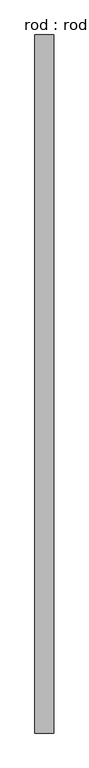
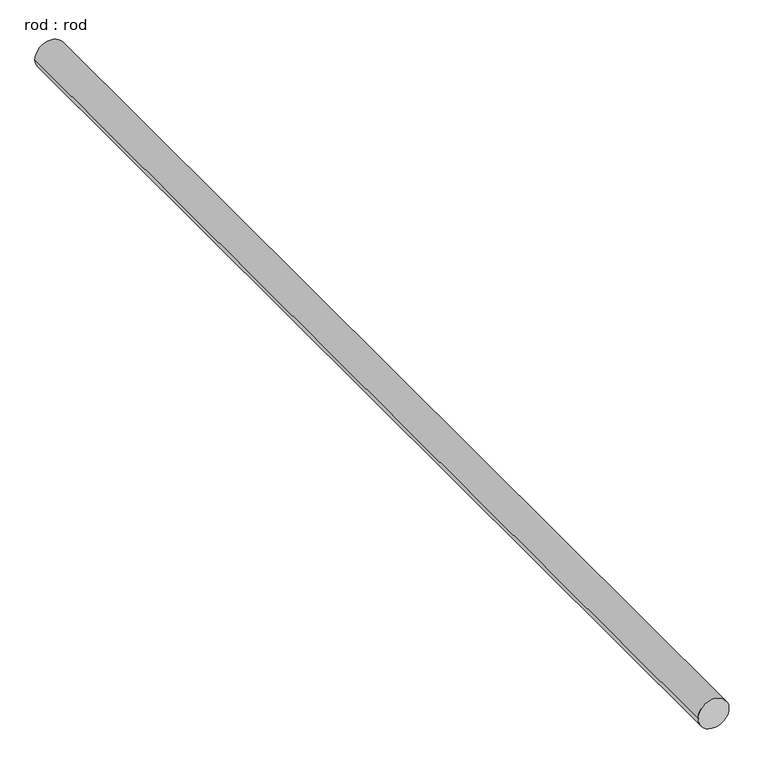
"""IFC4 building model written with IfcOpenShell, lengths in millimetres: proxy geometry, rod : rod."""

import ifcopenshell
import ifcopenshell.guid

model = None  # the IFC model being written
_history = None  # IfcOwnerHistory: only IFC2X3 demands one
_inside = {}  # id of a spatial element -> (the spatial element, [elements in it])
_under = {}  # id of a project, library or spatial element -> (it, [spatial elements below it])
_declared = {}  # id of a project -> (the project, [libraries it declares])
_typed = {}  # id of a type object -> (the type object, [elements of that type])
_made_of = {}  # id of a material, layer set ... -> (it, [elements and type objects made of it])


def new_model(schema):
    """Start an empty IFC model of exactly this schema.

    Asked for "IFC4X3", IfcOpenShell would pick the latest addendum, in which some entities
    have other attributes; the version numbers below select the first issue.
    IFC2X3 requires an IfcOwnerHistory on every rooted entity: one is made here for all.
    """
    global model, _history
    if schema == "IFC4X3":
        model = ifcopenshell.file(schema_version=(4, 3, 0, 0))
    else:
        model = ifcopenshell.file(schema=schema)
    _inside.clear()
    _under.clear()
    _declared.clear()
    _typed.clear()
    _made_of.clear()
    _history = None
    if model.schema == "IFC2X3":
        org = make("IfcOrganization", Name="unknown")
        user = make(
            "IfcPersonAndOrganization",
            ThePerson=make("IfcPerson", FamilyName="unknown"),
            TheOrganization=org,
        )
        app = make(
            "IfcApplication",
            ApplicationDeveloper=org,
            Version="unknown",
            ApplicationFullName="unknown",
            ApplicationIdentifier="unknown",
        )
        _history = make(
            "IfcOwnerHistory",
            OwningUser=user,
            OwningApplication=app,
            ChangeAction="ADDED",
            CreationDate=0,
        )
    return model


def make(cls, **values):
    """One entity of the class cls with the attributes given. An attribute that is None is left unset."""
    return model.create_entity(
        cls, **{name: value for name, value in values.items() if value is not None}
    )


def rooted(cls, **values):
    """An entity with a GlobalId (a new one), such as an element, a storey or a relation."""
    return make(cls, GlobalId=ifcopenshell.guid.new(), OwnerHistory=_history, **values)


def si_unit(unit_type, name, prefix=None):
    """IfcSIUnit, for example si_unit("LENGTHUNIT", "METRE", prefix="MILLI")."""
    return make("IfcSIUnit", UnitType=unit_type, Prefix=prefix, Name=name)


def assignment(units):
    """IfcUnitAssignment: the units of a project."""
    return None if units is None else make("IfcUnitAssignment", Units=units)


def point(xyz):
    """IfcCartesianPoint."""
    return None if xyz is None else make("IfcCartesianPoint", Coordinates=xyz)


def direction(xyz):
    """IfcDirection."""
    return None if xyz is None else make("IfcDirection", DirectionRatios=xyz)


def frame(location, z_axis=None, x_axis=None):
    """IfcAxis2Placement3D, a coordinate frame: its origin and axes. An axis left out is left unset."""
    return make(
        "IfcAxis2Placement3D",
        Location=point(location),
        Axis=direction(z_axis),
        RefDirection=direction(x_axis),
    )


def frame_2d(location, x_axis=None):
    """IfcAxis2Placement2D, a coordinate frame in the plane: its origin and x axis."""
    return make(
        "IfcAxis2Placement2D", Location=point(location), RefDirection=direction(x_axis)
    )


def origin():
    """The frame at (0, 0, 0) with its axes left unset."""
    return frame((0.0, 0.0, 0.0))


def place(relative_to, where):
    """IfcLocalPlacement: puts the frame where relative to a parent placement (None: the world)."""
    return make(
        "IfcLocalPlacement", PlacementRelTo=relative_to, RelativePlacement=where
    )


def context(
    kind, dimensions, precision=None, world=None, true_north=None, identifier=None
):
    """IfcGeometricRepresentationContext, for example the 3D "Model" context."""
    return make(
        "IfcGeometricRepresentationContext",
        ContextIdentifier=identifier,
        ContextType=kind,
        CoordinateSpaceDimension=dimensions,
        Precision=precision,
        WorldCoordinateSystem=world,
        TrueNorth=true_north,
    )


def project(units=None, contexts=None):
    """IfcProject with its units and contexts."""
    return rooted(
        "IfcProject",
        Name="project",
        RepresentationContexts=contexts,
        UnitsInContext=assignment(units),
    )


def spatial(cls, under=None, at=None, **own):
    """A site, building, storey or space (cls), placed at a placement, below another one or the project."""
    s = rooted(cls, ObjectPlacement=at, **own)
    if under is not None:
        _under.setdefault(under.id(), (under, []))[1].append(s)
    return s


def circle_curve(where, radius):
    """IfcCircle in the frame where."""
    return make("IfcCircle", Position=where, Radius=radius)


def trimmed(basis, trim1, trim2, sense, master):
    """IfcTrimmedCurve: the piece of a basis curve between two trims."""
    return make(
        "IfcTrimmedCurve",
        BasisCurve=basis,
        Trim1=trim1,
        Trim2=trim2,
        SenseAgreement=sense,
        MasterRepresentation=master,
    )


def segment(curve, same_sense, transition):
    """IfcCompositeCurveSegment."""
    return make(
        "IfcCompositeCurveSegment",
        Transition=transition,
        SameSense=same_sense,
        ParentCurve=curve,
    )


def composite_curve(segments, self_intersect=None):
    """IfcCompositeCurve: segments joined end to end."""
    return make("IfcCompositeCurve", Segments=segments, SelfIntersect=self_intersect)


def outline(outer, holes=None, kind="AREA"):
    """IfcArbitraryClosedProfileDef: a profile drawn as a closed curve; with holes, ...WithVoids."""
    if holes is None:
        return make("IfcArbitraryClosedProfileDef", ProfileType=kind, OuterCurve=outer)
    return make(
        "IfcArbitraryProfileDefWithVoids",
        ProfileType=kind,
        OuterCurve=outer,
        InnerCurves=holes,
    )


def extrude(swept, where, along, depth):
    """IfcExtrudedAreaSolid: the profile swept, set in the frame where, extruded along a direction by depth."""
    return make(
        "IfcExtrudedAreaSolid",
        SweptArea=swept,
        Position=where,
        ExtrudedDirection=direction(along),
        Depth=depth,
    )


def shape(context_of_items, identifier, shape_type, items):
    """IfcShapeRepresentation: the items that make up one representation, for example the "Body"."""
    return make(
        "IfcShapeRepresentation",
        ContextOfItems=context_of_items,
        RepresentationIdentifier=identifier,
        RepresentationType=shape_type,
        Items=items,
    )


def source(mapping_origin, context_of_items, identifier, shape_type, items):
    """IfcRepresentationMap: a shape defined once, which mapped items show again and again."""
    return make(
        "IfcRepresentationMap",
        MappingOrigin=mapping_origin,
        MappedRepresentation=shape(context_of_items, identifier, shape_type, items),
    )


def transform(
    local_origin,
    x_axis=None,
    y_axis=None,
    z_axis=None,
    scale=None,
    scale2=None,
    scale3=None,
    uniform=True,
):
    """IfcCartesianTransformationOperator3D, or its non-uniform kind. x_axis, y_axis, z_axis: its Axis1, 2, 3."""
    if uniform:
        return make(
            "IfcCartesianTransformationOperator3D",
            Axis1=direction(x_axis),
            Axis2=direction(y_axis),
            LocalOrigin=point(local_origin),
            Scale=scale,
            Axis3=direction(z_axis),
        )
    return make(
        "IfcCartesianTransformationOperator3DnonUniform",
        Axis1=direction(x_axis),
        Axis2=direction(y_axis),
        LocalOrigin=point(local_origin),
        Scale=scale,
        Axis3=direction(z_axis),
        Scale2=scale2,
        Scale3=scale3,
    )


def mapped(mapping_source, mapping_target):
    """IfcMappedItem: shows the shape of a source again, moved by a transform."""
    return make(
        "IfcMappedItem", MappingSource=mapping_source, MappingTarget=mapping_target
    )


def made_of(thing, what):
    """Note that an element or type object is made of a material, layer set ...; save() writes the relation."""
    if what is not None:
        _made_of.setdefault(what.id(), (what, []))[1].append(thing)
    return thing


def element(
    cls,
    number,
    at=None,
    inside=None,
    cuts=None,
    type_object=None,
    material=None,
    context=None,
    identifier="Body",
    shape_type=None,
    held_by="IfcProductDefinitionShape",
    body=None,
    shapes=None,
    **own,
):
    """One element of the class cls, such as IfcWall. Its Tag is "e" and its number.

    at: its placement. inside: the storey or other place that contains it. cuts: it is an
    opening in that element (IfcRelVoidsElement). A single representation is given by context,
    identifier, shape_type and body (its items); several are given by shapes. held_by: the class
    of the entity that holds the representations. save() writes the other relations.
    """
    e = rooted(cls, Tag="e%d" % number, ObjectPlacement=at, **own)
    if body is not None:
        shapes = [shape(context, identifier, shape_type, body)]
    if shapes is not None:
        e.Representation = make(held_by, Representations=shapes)
    if inside is not None:
        _inside.setdefault(inside.id(), (inside, []))[1].append(e)
    if cuts is not None:
        rooted(
            "IfcRelVoidsElement", RelatingBuildingElement=cuts, RelatedOpeningElement=e
        )
    if type_object is not None:
        _typed.setdefault(type_object.id(), (type_object, []))[1].append(e)
    return made_of(e, material)


def aggregate(whole, parts):
    """IfcRelAggregates: a whole, such as a stair, and the parts it consists of."""
    return rooted("IfcRelAggregates", RelatingObject=whole, RelatedObjects=parts)


def save(model, path):
    """Write the relations noted so far, then the file.

    IfcRelAggregates (storeys below a building ...), IfcRelContainedInSpatialStructure (elements
    in a storey), IfcRelDefinesByType, IfcRelAssociatesMaterial and IfcRelDeclares: one each for
    every whole, place, type object, material and project.
    """
    for whole, parts in _under.values():
        aggregate(whole, parts)
    for where, things in _inside.values():
        rooted(
            "IfcRelContainedInSpatialStructure",
            RelatedElements=things,
            RelatingStructure=where,
        )
    for kind, things in _typed.values():
        rooted("IfcRelDefinesByType", RelatedObjects=things, RelatingType=kind)
    for what, things in _made_of.values():
        rooted("IfcRelAssociatesMaterial", RelatedObjects=things, RelatingMaterial=what)
    for by, libraries in _declared.values():
        rooted("IfcRelDeclares", RelatingContext=by, RelatedDefinitions=libraries)
    model.write(path)


def rod_rod_d696530c(model_context):
    return source(origin(), model_context, "Body", "SweptSolid", [
        extrude(outline(composite_curve([segment(trimmed(circle_curve(frame_2d((0.0108462, 0.0)), 200.0), [point((0.0108462, 200.0))], [point((0.0108462, -200.0))], False, "CARTESIAN"), True, "CONTINUOUS"), segment(trimmed(circle_curve(frame_2d((0.0108462, 0.0)), 200.0), [point((0.0108462, -200.0))], [point((0.0108462, 200.0))], False, "CARTESIAN"), True, "CONTINUOUS")], self_intersect=False)), frame((0.0, -3367.5830404, 0.0), z_axis=(0.0, 1.0, 0.0), x_axis=(0.0, 0.0, 1.0)), (0.0, 0.0, 1.0), 14920.6233114),
    ])


if __name__ == "__main__":
    model = new_model("IFC4")
    model_context = context("Model", 3, world=origin())
    ifc_project = project(units=[si_unit("LENGTHUNIT", "METRE", prefix="MILLI")], contexts=[model_context])
    site = spatial("IfcSite", under=ifc_project)
    building = spatial("IfcBuilding", under=site)
    placement = place(None, origin())
    rod_rod_shape = rod_rod_d696530c(model_context)
    element("IfcBuildingElementProxy", 1, Name="rod : rod", ObjectType="rod : rod", at=placement, inside=building, context=model_context, shape_type="MappedRepresentation", body=[
        mapped(rod_rod_shape, transform((0.0, 0.0, 0.0), x_axis=(1.0, 0.0, 0.0), y_axis=(0.0, 1.0, 0.0), z_axis=(0.0, 0.0, 1.0))),
    ])
    save(model, "model.ifc")

# Revit data of these elements
# Type "rod : rod"
#   Default Elevation = 0
